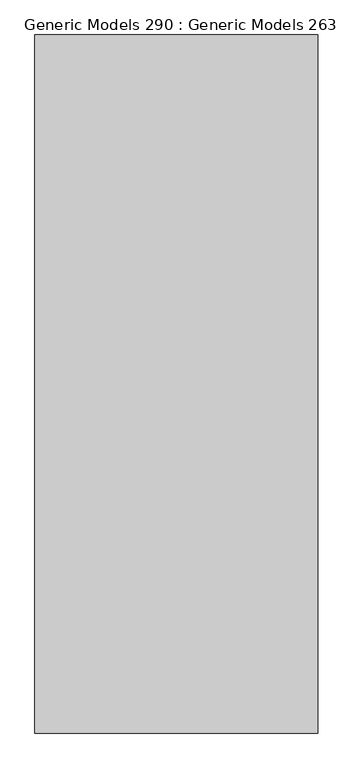
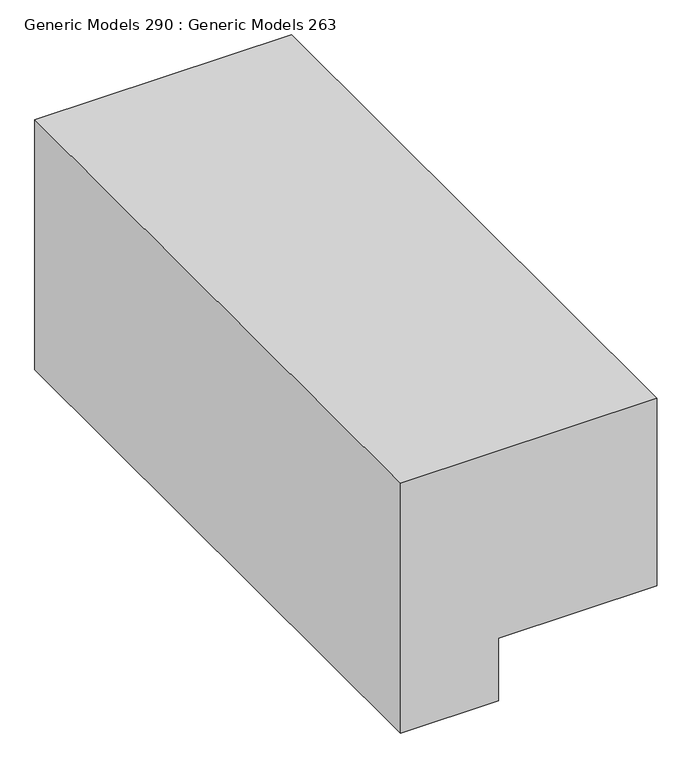
"""IFC4 building model written with IfcOpenShell, lengths in millimetres: proxy geometry, Generic Models 290 : Generic Models 263."""

import ifcopenshell
import ifcopenshell.guid

model = None  # the IFC model being written
_history = None  # IfcOwnerHistory: only IFC2X3 demands one
_inside = {}  # id of a spatial element -> (the spatial element, [elements in it])
_under = {}  # id of a project, library or spatial element -> (it, [spatial elements below it])
_declared = {}  # id of a project -> (the project, [libraries it declares])
_typed = {}  # id of a type object -> (the type object, [elements of that type])
_made_of = {}  # id of a material, layer set ... -> (it, [elements and type objects made of it])


def new_model(schema):
    """Start an empty IFC model of exactly this schema.

    Asked for "IFC4X3", IfcOpenShell would pick the latest addendum, in which some entities
    have other attributes; the version numbers below select the first issue.
    IFC2X3 requires an IfcOwnerHistory on every rooted entity: one is made here for all.
    """
    global model, _history
    if schema == "IFC4X3":
        model = ifcopenshell.file(schema_version=(4, 3, 0, 0))
    else:
        model = ifcopenshell.file(schema=schema)
    _inside.clear()
    _under.clear()
    _declared.clear()
    _typed.clear()
    _made_of.clear()
    _history = None
    if model.schema == "IFC2X3":
        org = make("IfcOrganization", Name="unknown")
        user = make(
            "IfcPersonAndOrganization",
            ThePerson=make("IfcPerson", FamilyName="unknown"),
            TheOrganization=org,
        )
        app = make(
            "IfcApplication",
            ApplicationDeveloper=org,
            Version="unknown",
            ApplicationFullName="unknown",
            ApplicationIdentifier="unknown",
        )
        _history = make(
            "IfcOwnerHistory",
            OwningUser=user,
            OwningApplication=app,
            ChangeAction="ADDED",
            CreationDate=0,
        )
    return model


def make(cls, **values):
    """One entity of the class cls with the attributes given. An attribute that is None is left unset."""
    return model.create_entity(
        cls, **{name: value for name, value in values.items() if value is not None}
    )


def rooted(cls, **values):
    """An entity with a GlobalId (a new one), such as an element, a storey or a relation."""
    return make(cls, GlobalId=ifcopenshell.guid.new(), OwnerHistory=_history, **values)


def si_unit(unit_type, name, prefix=None):
    """IfcSIUnit, for example si_unit("LENGTHUNIT", "METRE", prefix="MILLI")."""
    return make("IfcSIUnit", UnitType=unit_type, Prefix=prefix, Name=name)


def assignment(units):
    """IfcUnitAssignment: the units of a project."""
    return None if units is None else make("IfcUnitAssignment", Units=units)


def point(xyz):
    """IfcCartesianPoint."""
    return None if xyz is None else make("IfcCartesianPoint", Coordinates=xyz)


def direction(xyz):
    """IfcDirection."""
    return None if xyz is None else make("IfcDirection", DirectionRatios=xyz)


def frame(location, z_axis=None, x_axis=None):
    """IfcAxis2Placement3D, a coordinate frame: its origin and axes. An axis left out is left unset."""
    return make(
        "IfcAxis2Placement3D",
        Location=point(location),
        Axis=direction(z_axis),
        RefDirection=direction(x_axis),
    )


def origin():
    """The frame at (0, 0, 0) with its axes left unset."""
    return frame((0.0, 0.0, 0.0))


def place(relative_to, where):
    """IfcLocalPlacement: puts the frame where relative to a parent placement (None: the world)."""
    return make(
        "IfcLocalPlacement", PlacementRelTo=relative_to, RelativePlacement=where
    )


def context(
    kind, dimensions, precision=None, world=None, true_north=None, identifier=None
):
    """IfcGeometricRepresentationContext, for example the 3D "Model" context."""
    return make(
        "IfcGeometricRepresentationContext",
        ContextIdentifier=identifier,
        ContextType=kind,
        CoordinateSpaceDimension=dimensions,
        Precision=precision,
        WorldCoordinateSystem=world,
        TrueNorth=true_north,
    )


def project(units=None, contexts=None):
    """IfcProject with its units and contexts."""
    return rooted(
        "IfcProject",
        Name="project",
        RepresentationContexts=contexts,
        UnitsInContext=assignment(units),
    )


def spatial(cls, under=None, at=None, **own):
    """A site, building, storey or space (cls), placed at a placement, below another one or the project."""
    s = rooted(cls, ObjectPlacement=at, **own)
    if under is not None:
        _under.setdefault(under.id(), (under, []))[1].append(s)
    return s


def polyline(points):
    """IfcPolyline through the points."""
    return make("IfcPolyline", Points=[point(p) for p in points])


def outline(outer, holes=None, kind="AREA"):
    """IfcArbitraryClosedProfileDef: a profile drawn as a closed curve; with holes, ...WithVoids."""
    if holes is None:
        return make("IfcArbitraryClosedProfileDef", ProfileType=kind, OuterCurve=outer)
    return make(
        "IfcArbitraryProfileDefWithVoids",
        ProfileType=kind,
        OuterCurve=outer,
        InnerCurves=holes,
    )


def extrude(swept, where, along, depth):
    """IfcExtrudedAreaSolid: the profile swept, set in the frame where, extruded along a direction by depth."""
    return make(
        "IfcExtrudedAreaSolid",
        SweptArea=swept,
        Position=where,
        ExtrudedDirection=direction(along),
        Depth=depth,
    )


def shape(context_of_items, identifier, shape_type, items):
    """IfcShapeRepresentation: the items that make up one representation, for example the "Body"."""
    return make(
        "IfcShapeRepresentation",
        ContextOfItems=context_of_items,
        RepresentationIdentifier=identifier,
        RepresentationType=shape_type,
        Items=items,
    )


def source(mapping_origin, context_of_items, identifier, shape_type, items):
    """IfcRepresentationMap: a shape defined once, which mapped items show again and again."""
    return make(
        "IfcRepresentationMap",
        MappingOrigin=mapping_origin,
        MappedRepresentation=shape(context_of_items, identifier, shape_type, items),
    )


def transform(
    local_origin,
    x_axis=None,
    y_axis=None,
    z_axis=None,
    scale=None,
    scale2=None,
    scale3=None,
    uniform=True,
):
    """IfcCartesianTransformationOperator3D, or its non-uniform kind. x_axis, y_axis, z_axis: its Axis1, 2, 3."""
    if uniform:
        return make(
            "IfcCartesianTransformationOperator3D",
            Axis1=direction(x_axis),
            Axis2=direction(y_axis),
            LocalOrigin=point(local_origin),
            Scale=scale,
            Axis3=direction(z_axis),
        )
    return make(
        "IfcCartesianTransformationOperator3DnonUniform",
        Axis1=direction(x_axis),
        Axis2=direction(y_axis),
        LocalOrigin=point(local_origin),
        Scale=scale,
        Axis3=direction(z_axis),
        Scale2=scale2,
        Scale3=scale3,
    )


def mapped(mapping_source, mapping_target):
    """IfcMappedItem: shows the shape of a source again, moved by a transform."""
    return make(
        "IfcMappedItem", MappingSource=mapping_source, MappingTarget=mapping_target
    )


def made_of(thing, what):
    """Note that an element or type object is made of a material, layer set ...; save() writes the relation."""
    if what is not None:
        _made_of.setdefault(what.id(), (what, []))[1].append(thing)
    return thing


def element(
    cls,
    number,
    at=None,
    inside=None,
    cuts=None,
    type_object=None,
    material=None,
    context=None,
    identifier="Body",
    shape_type=None,
    held_by="IfcProductDefinitionShape",
    body=None,
    shapes=None,
    **own,
):
    """One element of the class cls, such as IfcWall. Its Tag is "e" and its number.

    at: its placement. inside: the storey or other place that contains it. cuts: it is an
    opening in that element (IfcRelVoidsElement). A single representation is given by context,
    identifier, shape_type and body (its items); several are given by shapes. held_by: the class
    of the entity that holds the representations. save() writes the other relations.
    """
    e = rooted(cls, Tag="e%d" % number, ObjectPlacement=at, **own)
    if body is not None:
        shapes = [shape(context, identifier, shape_type, body)]
    if shapes is not None:
        e.Representation = make(held_by, Representations=shapes)
    if inside is not None:
        _inside.setdefault(inside.id(), (inside, []))[1].append(e)
    if cuts is not None:
        rooted(
            "IfcRelVoidsElement", RelatingBuildingElement=cuts, RelatedOpeningElement=e
        )
    if type_object is not None:
        _typed.setdefault(type_object.id(), (type_object, []))[1].append(e)
    return made_of(e, material)


def aggregate(whole, parts):
    """IfcRelAggregates: a whole, such as a stair, and the parts it consists of."""
    return rooted("IfcRelAggregates", RelatingObject=whole, RelatedObjects=parts)


def save(model, path):
    """Write the relations noted so far, then the file.

    IfcRelAggregates (storeys below a building ...), IfcRelContainedInSpatialStructure (elements
    in a storey), IfcRelDefinesByType, IfcRelAssociatesMaterial and IfcRelDeclares: one each for
    every whole, place, type object, material and project.
    """
    for whole, parts in _under.values():
        aggregate(whole, parts)
    for where, things in _inside.values():
        rooted(
            "IfcRelContainedInSpatialStructure",
            RelatedElements=things,
            RelatingStructure=where,
        )
    for kind, things in _typed.values():
        rooted("IfcRelDefinesByType", RelatedObjects=things, RelatingType=kind)
    for what, things in _made_of.values():
        rooted("IfcRelAssociatesMaterial", RelatedObjects=things, RelatingMaterial=what)
    for by, libraries in _declared.values():
        rooted("IfcRelDeclares", RelatingContext=by, RelatedDefinitions=libraries)
    model.write(path)


def generic_models_290_generic_models_263_8c817db6(model_context):
    return source(origin(), model_context, "Body", "SweptSolid", [
        extrude(outline(polyline([(-381.0, 60490.3797726), (0.0, 60490.3797726), (0.0, 59996.6389907), (-508.0, 59996.6389907), (-508.0, 60185.5797726), (-381.0, 60185.5797726), (-381.0, 60490.3797726)])), frame((0.0, -94.4486541, 0.0), z_axis=(0.0, 1.0, 0.0), x_axis=(0.0, 0.0, 1.0)), (0.0, 0.0, 1.0), 1219.2),
    ])


if __name__ == "__main__":
    model = new_model("IFC4")
    model_context = context("Model", 3, world=origin())
    ifc_project = project(units=[si_unit("LENGTHUNIT", "METRE", prefix="MILLI")], contexts=[model_context])
    site = spatial("IfcSite", under=ifc_project)
    building = spatial("IfcBuilding", under=site)
    placement = place(None, origin())
    generic_models_290_generic_models_263_shape = generic_models_290_generic_models_263_8c817db6(model_context)
    element("IfcBuildingElementProxy", 1, Name="Generic Models 290 : Generic Models 263", ObjectType="Generic Models 290 : Generic Models 263", at=placement, inside=building, context=model_context, shape_type="MappedRepresentation", body=[
        mapped(generic_models_290_generic_models_263_shape, transform((0.0, 0.0, 0.0), x_axis=(1.0, 0.0, 0.0), y_axis=(0.0, 1.0, 0.0), z_axis=(0.0, 0.0, 1.0))),
    ])
    save(model, "model.ifc")

# Revit data of these elements
# Element 1 (IfcBuildingElementProxy, "Generic Models 290 : Generic Models 263")
#   Materials on its faces: "GRADED BACKFILL"
# Materials
#   "GRADED BACKFILL": class "Miscellaneous", colour RGB 128 97 77, transparency 0, Cost = 0
